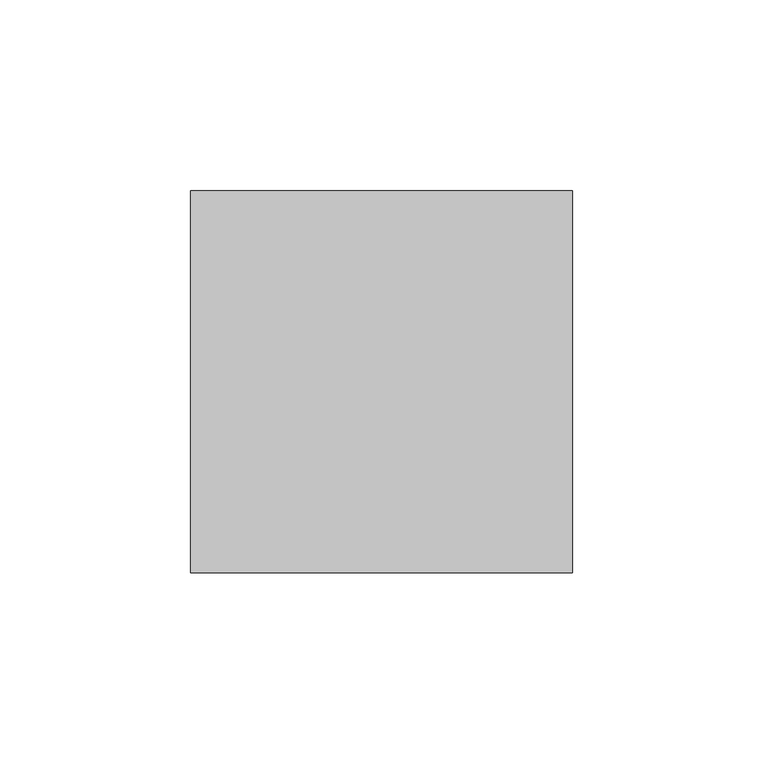
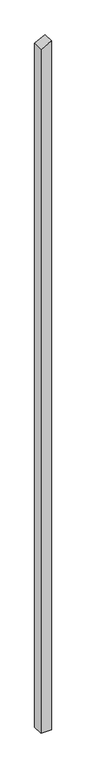
"""IFC4 building model written with IfcOpenShell, lengths in millimetres: column geometry, Holzstütze 159456 : Holzstütze 159456."""

from ifc_helpers import new_model, si_unit, frame, origin, place, context, project, spatial, polyline, outline, extrude, source, transform, mapped, element, save


def column_af8724ff(model_context):
    return source(origin(), model_context, "Body", "SweptSolid", [
        extrude(outline(polyline([(-500.0, 157297.7593015), (-500.0, 157397.7593015), (6396.6643707, 157397.7593015), (6345.7118258, 157297.7593015), (-500.0, 157297.7593015)])), frame((0.0, 47884.7962965, 0.0), z_axis=(0.0, 1.0, 0.0), x_axis=(0.0, 0.0, 1.0)), (0.0, 0.0, 1.0), 100.0),
    ])


if __name__ == "__main__":
    model = new_model("IFC4")
    model_context = context("Model", 3, world=origin())
    ifc_project = project(units=[si_unit("LENGTHUNIT", "METRE", prefix="MILLI")], contexts=[model_context])
    site = spatial("IfcSite", under=ifc_project)
    building = spatial("IfcBuilding", under=site)
    placement = place(None, origin())
    column_shape = column_af8724ff(model_context)
    element("IfcColumn", 1, ObjectType="Holzstütze 159456 : Holzstütze 159456", at=placement, inside=building, context=model_context, shape_type="MappedRepresentation", body=[
        mapped(column_shape, transform((0.0, 0.0, 0.0), x_axis=(1.0, 0.0, 0.0), y_axis=(0.0, 1.0, 0.0), z_axis=(0.0, 0.0, 1.0))),
    ])
    save(model, "model.ifc")

# Revit data of these elements
# Type "Holzstütze 159456 : Holzstütze 159456"
#   Abrechnungsart = "m"
#   Allright_Bauteil_ID = "0152St 0000143384"
#   Bezeichnung = "Holzstütze"
#   Codetext = "ST-HOLZ\\"
#   Gewerk = "Zimmer- und Holzbauarbeiten"
#   Material = "Holz"
#   Objektname = "Stütze"
#   NameOverride = "Holzstütze"
#   Reference = "Holzstütze"
#   Status = "NEW"
#   ThermalTransmittance = 0.0000 BTU/(h·ft²·°F)
#   Roll = 0.00°
#   Slope = 0.00°
#   2D Interaktion = yes
#   IsExternal = yes
#   LoadBearing = yes
# Element 1 (IfcColumn, "Holzstütze 159456 : Holzstütze 159456")
#   Materials on its faces: "holzschalung"
# Materials
#   "holzschalung": class "Unassigned", colour RGB 128 128 128, transparency 0
